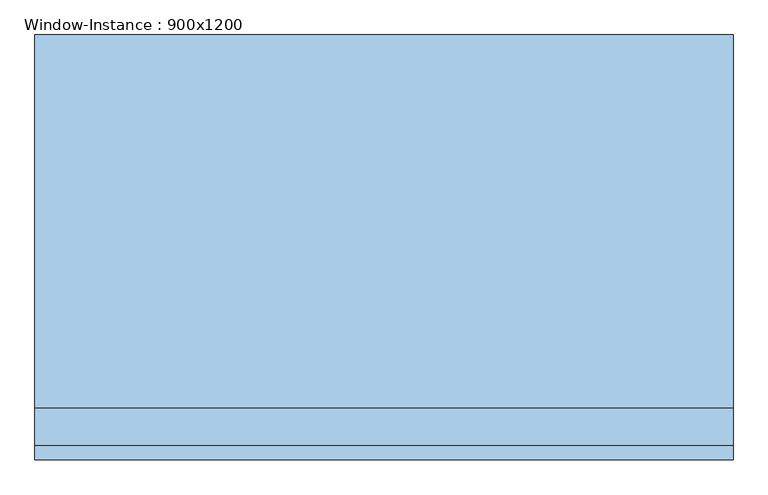
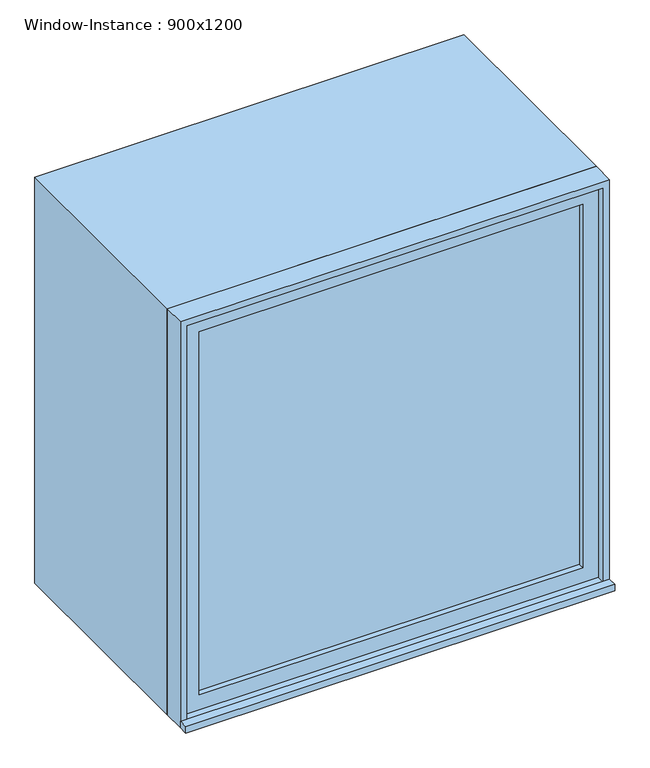
"""IFC4 building model written with IfcOpenShell, lengths in millimetres: window geometry, Window-Instance : 900x1200."""

from ifc_helpers import new_model, si_unit, frame, origin, place, context, project, spatial, polyline, outline, extrude, source, transform, mapped, element, save


def window_instance_900x1200_19ddbf74(model_context):
    return source(origin(), model_context, "Body", "SweptSolid", [
        extrude(outline(polyline([(-638.1, -377.9), (-638.1, -352.5), (561.9, -352.5), (561.9, -377.9), (-638.1, -377.9)])), frame((0.0, 0.0, 900.0), z_axis=(0.0, 0.0, 1.0), x_axis=(1.0, 0.0, 0.0)), (0.0, 0.0, 1.0), 19.05),
        extrude(outline(polyline([(498.4, -303.925), (498.4, -316.625), (-574.6, -316.625), (-574.6, -303.925), (498.4, -303.925)])), frame((0.0, 0.0, 963.5), z_axis=(0.0, 0.0, 1.0), x_axis=(1.0, 0.0, 0.0)), (0.0, 0.0, 1.0), 1073.0),
        extrude(outline(polyline([(2080.95, -619.05), (919.05, -619.05), (919.05, 542.85), (2080.95, 542.85), (2080.95, -619.05)]), holes=[polyline([(2036.5, -574.6), (2036.5, 498.4), (963.5, 498.4), (963.5, -574.6), (2036.5, -574.6)])]), frame((0.0, -332.5, 0.0), z_axis=(0.0, 1.0, 0.0), x_axis=(0.0, 0.0, 1.0)), (0.0, 0.0, 1.0), 44.45),
        extrude(outline(polyline([(2100.0, -638.1), (900.0, -638.1), (900.0, 561.9), (2100.0, 561.9), (2100.0, -638.1)]), holes=[polyline([(2068.25, -606.35), (2068.25, 530.15), (931.75, 530.15), (931.75, -606.35), (2068.25, -606.35)])]), frame((0.0, -288.05, 0.0), z_axis=(0.0, 1.0, 0.0), x_axis=(0.0, 0.0, 1.0)), (0.0, 0.0, 1.0), 640.55),
        extrude(outline(polyline([(2100.0, 561.9), (2100.0, -638.1), (900.0, -638.1), (900.0, 561.9), (2100.0, 561.9)]), holes=[polyline([(2080.95, 542.85), (919.05, 542.85), (919.05, -619.05), (2080.95, -619.05), (2080.95, 542.85)])]), frame((0.0, -352.5, 0.0), z_axis=(0.0, 1.0, 0.0), x_axis=(0.0, 0.0, 1.0)), (0.0, 0.0, 1.0), 64.45),
    ])


if __name__ == "__main__":
    model = new_model("IFC4")
    model_context = context("Model", 3, world=origin())
    ifc_project = project(units=[si_unit("LENGTHUNIT", "METRE", prefix="MILLI")], contexts=[model_context])
    site = spatial("IfcSite", under=ifc_project)
    building = spatial("IfcBuilding", under=site)
    placement = place(None, origin())
    window_instance_900x1200_shape = window_instance_900x1200_19ddbf74(model_context)
    element("IfcWindow", 1, ObjectType="Window-Instance : 900x1200", at=placement, inside=building, context=model_context, shape_type="MappedRepresentation", body=[
        mapped(window_instance_900x1200_shape, transform((0.0, 0.0, 0.0), x_axis=(1.0, 0.0, 0.0), y_axis=(0.0, 1.0, 0.0), z_axis=(0.0, 0.0, 1.0))),
    ])
    save(model, "model.ifc")

# Revit data of these elements
# Type "Window-Instance : 900x1200"
#   Type Mark = "10"
#   Construction Type Id = "GSP4R"
#   Assembly Code = "B2020100"
#   Analytic Construction = "1/8 in Pilkington single glazing"
#   Visual Light Transmittance = 0.9
#   Thermal Resistance (R) = 0.149095 (m²·K)/W
#   Solar Heat Gain Coefficient = 0.86
#   Heat Transfer Coefficient (U) = 6.70716 W/(m²·K)
#   Height [instance default] = 1200 mm
#   Default Sill Height = 900 mm
#   Width [instance default] = 600 mm
#   Window Inset = 20 mm
#   Glass Pane Material = none
#   Sash Material = none
#   Wall Closure = (empty or 0)
# Element 1 (IfcWindow, "Window-Instance : 900x1200")
#   Width = 1200 mm
